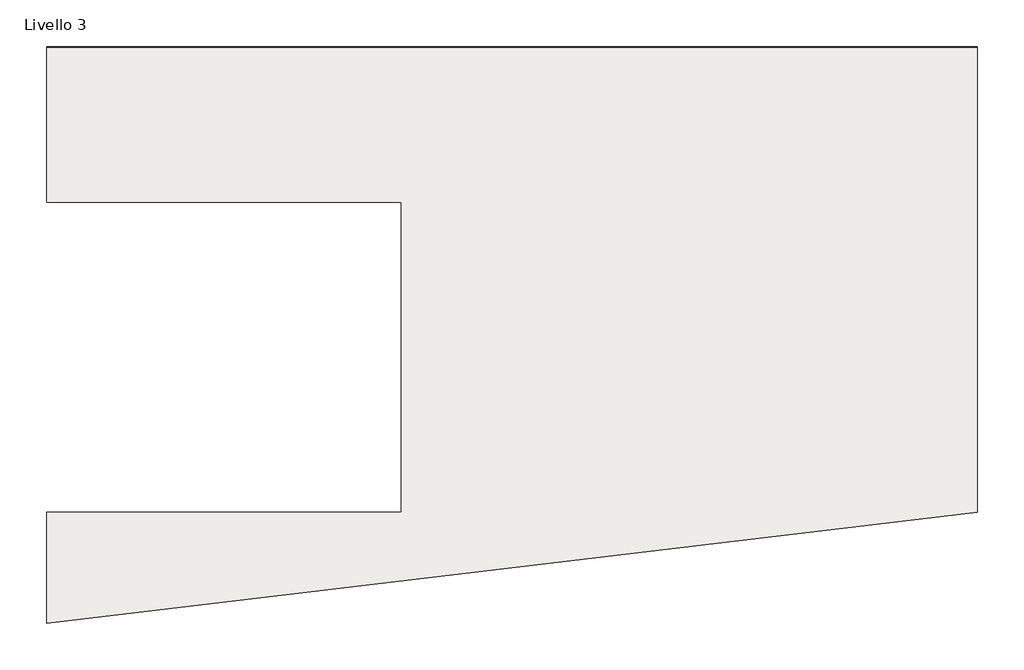
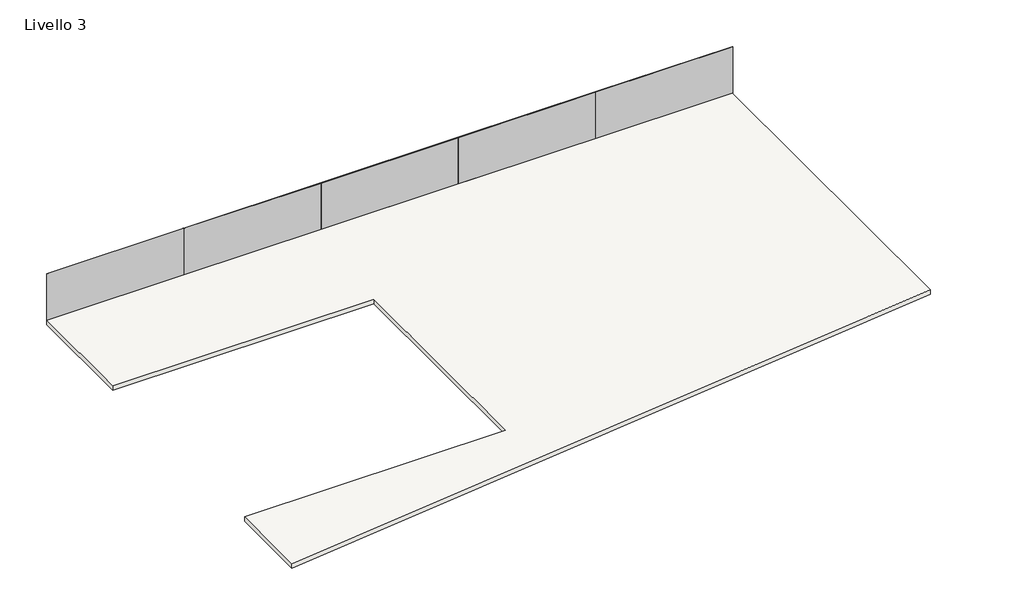
# One storey: 5 plates, 1 slab.
"""IFC4 building model written with IfcOpenShell, lengths in millimetres."""

import ifcopenshell
import ifcopenshell.guid

model = None  # the IFC model being written
_history = None  # IfcOwnerHistory: only IFC2X3 demands one
_inside = {}  # id of a spatial element -> (the spatial element, [elements in it])
_under = {}  # id of a project, library or spatial element -> (it, [spatial elements below it])
_declared = {}  # id of a project -> (the project, [libraries it declares])
_typed = {}  # id of a type object -> (the type object, [elements of that type])
_made_of = {}  # id of a material, layer set ... -> (it, [elements and type objects made of it])


def new_model(schema):
    """Start an empty IFC model of exactly this schema.

    Asked for "IFC4X3", IfcOpenShell would pick the latest addendum, in which some entities
    have other attributes; the version numbers below select the first issue.
    IFC2X3 requires an IfcOwnerHistory on every rooted entity: one is made here for all.
    """
    global model, _history
    if schema == "IFC4X3":
        model = ifcopenshell.file(schema_version=(4, 3, 0, 0))
    else:
        model = ifcopenshell.file(schema=schema)
    _inside.clear()
    _under.clear()
    _declared.clear()
    _typed.clear()
    _made_of.clear()
    _history = None
    if model.schema == "IFC2X3":
        org = make("IfcOrganization", Name="unknown")
        user = make(
            "IfcPersonAndOrganization",
            ThePerson=make("IfcPerson", FamilyName="unknown"),
            TheOrganization=org,
        )
        app = make(
            "IfcApplication",
            ApplicationDeveloper=org,
            Version="unknown",
            ApplicationFullName="unknown",
            ApplicationIdentifier="unknown",
        )
        _history = make(
            "IfcOwnerHistory",
            OwningUser=user,
            OwningApplication=app,
            ChangeAction="ADDED",
            CreationDate=0,
        )
    return model


def make(cls, **values):
    """One entity of the class cls with the attributes given. An attribute that is None is left unset."""
    return model.create_entity(
        cls, **{name: value for name, value in values.items() if value is not None}
    )


def rooted(cls, **values):
    """An entity with a GlobalId (a new one), such as an element, a storey or a relation."""
    return make(cls, GlobalId=ifcopenshell.guid.new(), OwnerHistory=_history, **values)


def si_unit(unit_type, name, prefix=None):
    """IfcSIUnit, for example si_unit("LENGTHUNIT", "METRE", prefix="MILLI")."""
    return make("IfcSIUnit", UnitType=unit_type, Prefix=prefix, Name=name)


def assignment(units):
    """IfcUnitAssignment: the units of a project."""
    return None if units is None else make("IfcUnitAssignment", Units=units)


def point(xyz):
    """IfcCartesianPoint."""
    return None if xyz is None else make("IfcCartesianPoint", Coordinates=xyz)


def direction(xyz):
    """IfcDirection."""
    return None if xyz is None else make("IfcDirection", DirectionRatios=xyz)


def frame(location, z_axis=None, x_axis=None):
    """IfcAxis2Placement3D, a coordinate frame: its origin and axes. An axis left out is left unset."""
    return make(
        "IfcAxis2Placement3D",
        Location=point(location),
        Axis=direction(z_axis),
        RefDirection=direction(x_axis),
    )


def origin():
    """The frame at (0, 0, 0) with its axes left unset."""
    return frame((0.0, 0.0, 0.0))


def origin_with_axes():
    """The frame at (0, 0, 0) with the z axis (0, 0, 1) and the x axis (1, 0, 0) written out."""
    return frame((0.0, 0.0, 0.0), z_axis=(0.0, 0.0, 1.0), x_axis=(1.0, 0.0, 0.0))


def place(relative_to, where):
    """IfcLocalPlacement: puts the frame where relative to a parent placement (None: the world)."""
    return make(
        "IfcLocalPlacement", PlacementRelTo=relative_to, RelativePlacement=where
    )


def context(
    kind, dimensions, precision=None, world=None, true_north=None, identifier=None
):
    """IfcGeometricRepresentationContext, for example the 3D "Model" context."""
    return make(
        "IfcGeometricRepresentationContext",
        ContextIdentifier=identifier,
        ContextType=kind,
        CoordinateSpaceDimension=dimensions,
        Precision=precision,
        WorldCoordinateSystem=world,
        TrueNorth=true_north,
    )


def project(units=None, contexts=None):
    """IfcProject with its units and contexts."""
    return rooted(
        "IfcProject",
        Name="project",
        RepresentationContexts=contexts,
        UnitsInContext=assignment(units),
    )


def spatial(cls, under=None, at=None, **own):
    """A site, building, storey or space (cls), placed at a placement, below another one or the project."""
    s = rooted(cls, ObjectPlacement=at, **own)
    if under is not None:
        _under.setdefault(under.id(), (under, []))[1].append(s)
    return s


def polyline(points):
    """IfcPolyline through the points."""
    return make("IfcPolyline", Points=[point(p) for p in points])


def outline(outer, holes=None, kind="AREA"):
    """IfcArbitraryClosedProfileDef: a profile drawn as a closed curve; with holes, ...WithVoids."""
    if holes is None:
        return make("IfcArbitraryClosedProfileDef", ProfileType=kind, OuterCurve=outer)
    return make(
        "IfcArbitraryProfileDefWithVoids",
        ProfileType=kind,
        OuterCurve=outer,
        InnerCurves=holes,
    )


def extrude(swept, where, along, depth):
    """IfcExtrudedAreaSolid: the profile swept, set in the frame where, extruded along a direction by depth."""
    return make(
        "IfcExtrudedAreaSolid",
        SweptArea=swept,
        Position=where,
        ExtrudedDirection=direction(along),
        Depth=depth,
    )


def shape(context_of_items, identifier, shape_type, items):
    """IfcShapeRepresentation: the items that make up one representation, for example the "Body"."""
    return make(
        "IfcShapeRepresentation",
        ContextOfItems=context_of_items,
        RepresentationIdentifier=identifier,
        RepresentationType=shape_type,
        Items=items,
    )


def source(mapping_origin, context_of_items, identifier, shape_type, items):
    """IfcRepresentationMap: a shape defined once, which mapped items show again and again."""
    return make(
        "IfcRepresentationMap",
        MappingOrigin=mapping_origin,
        MappedRepresentation=shape(context_of_items, identifier, shape_type, items),
    )


def transform(
    local_origin,
    x_axis=None,
    y_axis=None,
    z_axis=None,
    scale=None,
    scale2=None,
    scale3=None,
    uniform=True,
):
    """IfcCartesianTransformationOperator3D, or its non-uniform kind. x_axis, y_axis, z_axis: its Axis1, 2, 3."""
    if uniform:
        return make(
            "IfcCartesianTransformationOperator3D",
            Axis1=direction(x_axis),
            Axis2=direction(y_axis),
            LocalOrigin=point(local_origin),
            Scale=scale,
            Axis3=direction(z_axis),
        )
    return make(
        "IfcCartesianTransformationOperator3DnonUniform",
        Axis1=direction(x_axis),
        Axis2=direction(y_axis),
        LocalOrigin=point(local_origin),
        Scale=scale,
        Axis3=direction(z_axis),
        Scale2=scale2,
        Scale3=scale3,
    )


def mapped(mapping_source, mapping_target):
    """IfcMappedItem: shows the shape of a source again, moved by a transform."""
    return make(
        "IfcMappedItem", MappingSource=mapping_source, MappingTarget=mapping_target
    )


def made_of(thing, what):
    """Note that an element or type object is made of a material, layer set ...; save() writes the relation."""
    if what is not None:
        _made_of.setdefault(what.id(), (what, []))[1].append(thing)
    return thing


def element(
    cls,
    number,
    at=None,
    inside=None,
    cuts=None,
    type_object=None,
    material=None,
    context=None,
    identifier="Body",
    shape_type=None,
    held_by="IfcProductDefinitionShape",
    body=None,
    shapes=None,
    **own,
):
    """One element of the class cls, such as IfcWall. Its Tag is "e" and its number.

    at: its placement. inside: the storey or other place that contains it. cuts: it is an
    opening in that element (IfcRelVoidsElement). A single representation is given by context,
    identifier, shape_type and body (its items); several are given by shapes. held_by: the class
    of the entity that holds the representations. save() writes the other relations.
    """
    e = rooted(cls, Tag="e%d" % number, ObjectPlacement=at, **own)
    if body is not None:
        shapes = [shape(context, identifier, shape_type, body)]
    if shapes is not None:
        e.Representation = make(held_by, Representations=shapes)
    if inside is not None:
        _inside.setdefault(inside.id(), (inside, []))[1].append(e)
    if cuts is not None:
        rooted(
            "IfcRelVoidsElement", RelatingBuildingElement=cuts, RelatedOpeningElement=e
        )
    if type_object is not None:
        _typed.setdefault(type_object.id(), (type_object, []))[1].append(e)
    return made_of(e, material)


def aggregate(whole, parts):
    """IfcRelAggregates: a whole, such as a stair, and the parts it consists of."""
    return rooted("IfcRelAggregates", RelatingObject=whole, RelatedObjects=parts)


def save(model, path):
    """Write the relations noted so far, then the file.

    IfcRelAggregates (storeys below a building ...), IfcRelContainedInSpatialStructure (elements
    in a storey), IfcRelDefinesByType, IfcRelAssociatesMaterial and IfcRelDeclares: one each for
    every whole, place, type object, material and project.
    """
    for whole, parts in _under.values():
        aggregate(whole, parts)
    for where, things in _inside.values():
        rooted(
            "IfcRelContainedInSpatialStructure",
            RelatedElements=things,
            RelatingStructure=where,
        )
    for kind, things in _typed.values():
        rooted("IfcRelDefinesByType", RelatedObjects=things, RelatingType=kind)
    for what, things in _made_of.values():
        rooted("IfcRelAssociatesMaterial", RelatedObjects=things, RelatingMaterial=what)
    for by, libraries in _declared.values():
        rooted("IfcRelDeclares", RelatingContext=by, RelatedDefinitions=libraries)
    model.write(path)


def pannello_sistema_vetrato_29ff3466(model_context):
    return source(origin(), model_context, "Body", "SweptSolid", [
        extrude(outline(polyline([(4200.0000001, -15.0), (-4200.0000001, -15.0), (-4200.0000001, 15.0), (4200.0000001, 15.0), (4200.0000001, -15.0)])), origin_with_axes(), (0.0, 0.0, 1.0), 3000.0),
    ])


model = new_model("IFC4")

# Units and contexts
model_context = context("Model", 3, world=origin())
ifc_project = project(units=[si_unit("LENGTHUNIT", "METRE", prefix="MILLI")], contexts=[model_context])

# Site, building, storey
site = spatial("IfcSite", under=ifc_project)
building = spatial("IfcBuilding", under=site)
storey = spatial("IfcBuildingStorey", under=building, Name="Livello 3", Elevation=9000.0)

# Plates
placement = place(None, origin())
pannello_sistema_vetrato_shape = pannello_sistema_vetrato_29ff3466(model_context)
element("IfcPlate", 1, ObjectType="Pannello sistema : Vetrato", at=placement, inside=storey, context=model_context, shape_type="MappedRepresentation", body=[
    mapped(pannello_sistema_vetrato_shape, transform((-20934.9893485, 13197.4454735, 9000.0), x_axis=(1.0, 0.0, 0.0), y_axis=(0.0, 1.0, 0.0), z_axis=(0.0, 0.0, 1.0))),
])
element("IfcPlate", 2, ObjectType="Pannello sistema : Vetrato", at=placement, inside=storey, context=model_context, shape_type="MappedRepresentation", body=[
    mapped(pannello_sistema_vetrato_shape, transform((-12534.9893485, 13197.4454735, 9000.0), x_axis=(1.0, 0.0, 0.0), y_axis=(0.0, 1.0, 0.0), z_axis=(0.0, 0.0, 1.0))),
])
element("IfcPlate", 3, ObjectType="Pannello sistema : Vetrato", at=placement, inside=storey, context=model_context, shape_type="MappedRepresentation", body=[
    mapped(pannello_sistema_vetrato_shape, transform((-4134.9893486, 13197.4454735, 9000.0), x_axis=(1.0, 0.0, 0.0), y_axis=(0.0, 1.0, 0.0), z_axis=(0.0, 0.0, 1.0))),
])
element("IfcPlate", 4, ObjectType="Pannello sistema : Vetrato", at=placement, inside=storey, context=model_context, shape_type="MappedRepresentation", body=[
    mapped(pannello_sistema_vetrato_shape, transform((4265.0106513, 13197.4454735, 9000.0), x_axis=(1.0, 0.0, 0.0), y_axis=(0.0, 1.0, 0.0), z_axis=(0.0, 0.0, 1.0))),
])
element("IfcPlate", 5, ObjectType="Pannello sistema : Vetrato", at=placement, inside=storey, context=model_context, shape_type="MappedRepresentation", body=[
    mapped(pannello_sistema_vetrato_shape, transform((12665.0106513, 13197.4454735, 9000.0), x_axis=(1.0, 0.0, 0.0), y_axis=(0.0, 1.0, 0.0), z_axis=(0.0, 0.0, 1.0))),
])

# Slab
element("IfcSlab", 6, ObjectType="Latero Cementizio - 30 cm", at=placement, inside=storey, context=model_context, shape_type="SweptSolid", body=[
    extrude(outline(polyline([(-25134.9893486, -7802.5545265), (-9134.9893486, -7802.5545265), (-9134.9893486, 6197.4454735), (-25134.9893486, 6197.4454735), (-25134.9893486, 13197.4454735), (16865.0106514, 13197.4454735), (16865.0106514, -7802.5545265), (-25134.9893486, -12802.5545265), (-25134.9893486, -7802.5545265)])), frame((0.0, 0.0, 8700.0), z_axis=(0.0, 0.0, 1.0), x_axis=(1.0, 0.0, 0.0)), (0.0, 0.0, 1.0), 300.0),
])

save(model, "model.ifc")

# Revit data of these elements
# Type "Pannello sistema : Vetrato"
#   Construction Type Id = "GSP4R"
#   Analytic Construction = "Vetrata singola Pilkington 1/8 in"
#   Visual Light Transmittance = 0.9
#   Solar Heat Gain Coefficient = 0.86
#   Heat Transfer Coefficient (U) = 6.7069 W/(m²·K)
# Type "Latero Cementizio - 30 cm"
#   Keynote = "S/3"
#   Function = 0
#   Layers, outside or top first: 0.02 m "Ceramica bianca" (function 4); 0.065 m "Sabbia e Calcestruzzo" (function 2); 0.04 m "Calcestruzzo" (function 1); 0.16 m "Laterizio (2)" (function 1); 0.015 m "Intonaco - Bianco" (function 5)
# Elements 1, 2, 3, 4, 5 (IfcPlate, "Pannello sistema : Vetrato")
#   Phase Created = Stato di Progetto
#   Materials on its faces: "Default - Vetro"
# Element 6 (IfcSlab, "Latero Cementizio - 30 cm")
#   built-in parameter 1001955 = 1.5708 (stored number, unit not read)
#   Height Offset From Level = 0.00 m
#   Phase Created = Stato di Progetto
#   Materials on its faces: "Intonaco - Bianco", "Ceramica bianca"
# Materials
#   "Ceramica bianca": class "Ceramica", colour RGB 210 210 210, transparency 0, Description = "Finitura interna - Piastrelle di ceramica incollate", Cost = 0
#   "Sabbia e Calcestruzzo": class "Calcestruzzo", colour RGB 127 127 127, transparency 0, Description = "Magrone - Sabbia e cemento", Cost = 0
#   "Calcestruzzo": class "Calcestruzzo", colour RGB 192 192 192, transparency 0, Description = "Calcestruzzo - Cemento Portland", Cost = 0
#   "Laterizio (2)": class "Mattone", colour RGB 255 128 64, transparency 0, Description = "Pignatta h 16 cm", Cost = 0
#   "Intonaco - Bianco": class "Intonaco", colour RGB 249 249 249, transparency 0, Description = "Verniciatura", Cost = 0
#   "Default - Vetro": class "Vetro", colour RGB 208 208 208, transparency 0.7, Cost = 0
